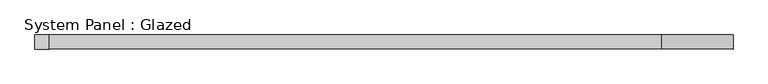
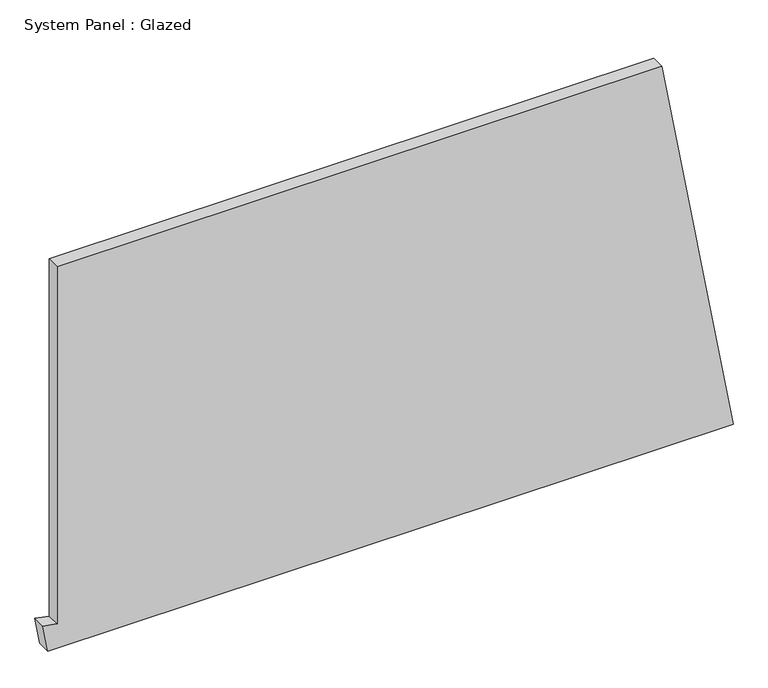
"""IFC4 building model written with IfcOpenShell, lengths in millimetres: plate geometry, System Panel : Glazed."""

from ifc_helpers import new_model, si_unit, frame, origin, place, context, project, spatial, polyline, outline, extrude, source, transform, mapped, element, save


def system_panel_glazed_1798d0a9(model_context):
    return source(origin(), model_context, "Body", "SweptSolid", [
        extrude(outline(polyline([(0.0, -611.2128166), (0.0, 620.1390218), (725.0, 492.3019608), (725.0, -594.7592156), (46.2818207, -594.7592156), (50.6230251, -620.1390218), (0.0, -611.2128166)])), frame((0.0, -49.5, 0.0), z_axis=(0.0, 1.0, 0.0), x_axis=(0.0, 0.0, 1.0)), (0.0, 0.0, 1.0), 25.0),
    ])


if __name__ == "__main__":
    model = new_model("IFC4")
    model_context = context("Model", 3, world=origin())
    ifc_project = project(units=[si_unit("LENGTHUNIT", "METRE", prefix="MILLI")], contexts=[model_context])
    site = spatial("IfcSite", under=ifc_project)
    building = spatial("IfcBuilding", under=site)
    placement = place(None, origin())
    system_panel_glazed_shape = system_panel_glazed_1798d0a9(model_context)
    element("IfcPlate", 1, ObjectType="System Panel : Glazed", at=placement, inside=building, context=model_context, shape_type="MappedRepresentation", body=[
        mapped(system_panel_glazed_shape, transform((0.0, 0.0, 0.0), x_axis=(1.0, 0.0, 0.0), y_axis=(0.0, 1.0, 0.0), z_axis=(0.0, 0.0, 1.0))),
    ])
    save(model, "model.ifc")

# Revit data of these elements
# Project information
#   Project Issue Date = "Issue Date"
#   Project Status = "Project Status"
#   Client Name = "Owner"
#   Project Address = "Enter address here"
#   Project Name = "Project Name"
#   Project Number = "0001"
# Type "System Panel : Glazed"
#   Construction Type Id = "GSP4R"
#   Analytic Construction = "1/8 in Pilkington single glazing"
#   Visual Light Transmittance = 0.9
#   Solar Heat Gain Coefficient = 0.86
#   Heat Transfer Coefficient (U) = 6.7069 W/(m²·K)
#   Define Thermal Properties by = 1
# Element 1 (IfcPlate, "System Panel : Glazed")
#   Materials on its faces: "Glass"
# Materials
#   "Glass": class "Glass", colour RGB 0 128 192, transparency 0.9, Description = "Soda Lime Glass", Cost = 0
